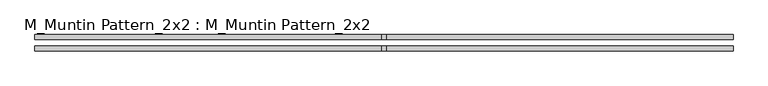
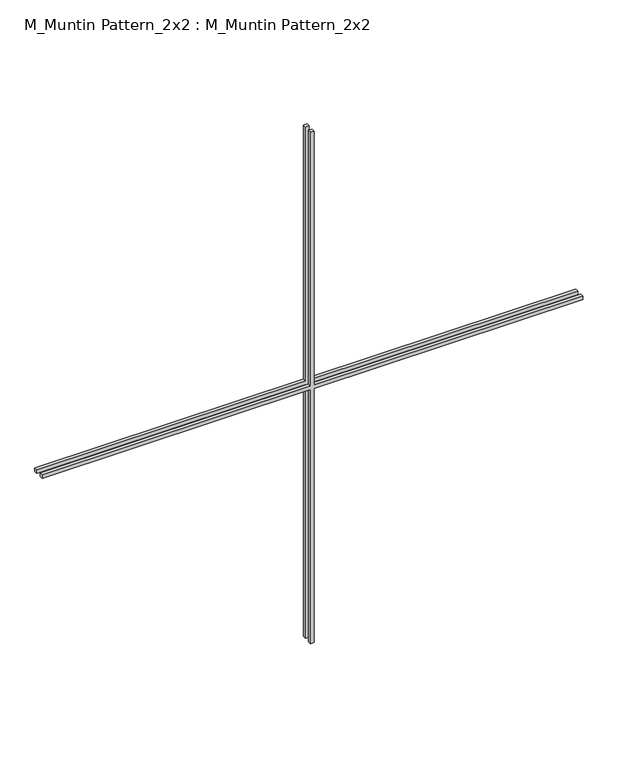
"""IFC4 building model written with IfcOpenShell, lengths in millimetres: proxy geometry, M_Muntin Pattern_2x2 : M_Muntin Pattern_2x2."""

from ifc_helpers import new_model, si_unit, frame, origin, place, context, project, spatial, polyline, outline, extrude, source, transform, mapped, element, save


def m_muntin_pattern_2x2_m_muntin_pattern_2x2_6261bc45(model_context):
    return source(origin(), model_context, "Body", "SweptSolid", [
        extrude(outline(polyline([(968.25, -6.35), (968.25, -961.9), (955.55, -961.9), (955.55, -6.35), (0.0, -6.35), (0.0, 6.35), (955.55, 6.35), (955.55, 961.9), (968.25, 961.9), (968.25, 6.35), (1923.8, 6.35), (1923.8, -6.35), (968.25, -6.35)])), frame((0.0, -22.225, 0.0), z_axis=(0.0, 1.0, 0.0), x_axis=(0.0, 0.0, 1.0)), (0.0, 0.0, 1.0), 12.7),
        extrude(outline(polyline([(968.25, -6.35), (968.25, -961.9), (955.55, -961.9), (955.55, -6.35), (0.0, -6.35), (0.0, 6.35), (955.55, 6.35), (955.55, 961.9), (968.25, 961.9), (968.25, 6.35), (1923.8, 6.35), (1923.8, -6.35), (968.25, -6.35)])), frame((0.0, 9.525, 0.0), z_axis=(0.0, 1.0, 0.0), x_axis=(0.0, 0.0, 1.0)), (0.0, 0.0, 1.0), 12.7),
    ])


if __name__ == "__main__":
    model = new_model("IFC4")
    model_context = context("Model", 3, world=origin())
    ifc_project = project(units=[si_unit("LENGTHUNIT", "METRE", prefix="MILLI")], contexts=[model_context])
    site = spatial("IfcSite", under=ifc_project)
    building = spatial("IfcBuilding", under=site)
    placement = place(None, origin())
    m_muntin_pattern_2x2_m_muntin_pattern_2x2_shape = m_muntin_pattern_2x2_m_muntin_pattern_2x2_6261bc45(model_context)
    element("IfcBuildingElementProxy", 1, Name="M_Muntin Pattern_2x2 : M_Muntin Pattern_2x2", ObjectType="M_Muntin Pattern_2x2 : M_Muntin Pattern_2x2", at=placement, inside=building, context=model_context, shape_type="MappedRepresentation", body=[
        mapped(m_muntin_pattern_2x2_m_muntin_pattern_2x2_shape, transform((0.0, 0.0, 0.0), x_axis=(1.0, 0.0, 0.0), y_axis=(0.0, 1.0, 0.0), z_axis=(0.0, 0.0, 1.0))),
    ])
    save(model, "model.ifc")

# Revit data of these elements
# Type "M_Muntin Pattern_2x2 : M_Muntin Pattern_2x2"
#   Width [instance default] = 1200 mm
#   Thickness = 12.7 mm
#   Height [instance default] = 1200 mm
#   Distance = 19.05 mm
#   Interior Material [instance default] = none
#   Exterior Material [instance default] = none
#   Default Elevation = 0
# Element 1 (IfcBuildingElementProxy, "M_Muntin Pattern_2x2 : M_Muntin Pattern_2x2")
#   Width = 1923.8 mm
#   Height = 1923.8 mm
#   Interior Material = Wood - Stained
#   Exterior Material = Clad - White
#   Materials on its faces: "Clad - White", "Wood - Stained"
# Materials
#   "Clad - White": class "Wood", colour RGB 245 245 243, transparency 0, Cost = 0
#   "Wood - Stained": class "Wood", colour RGB 173 132 96, transparency 0, Cost = 0
